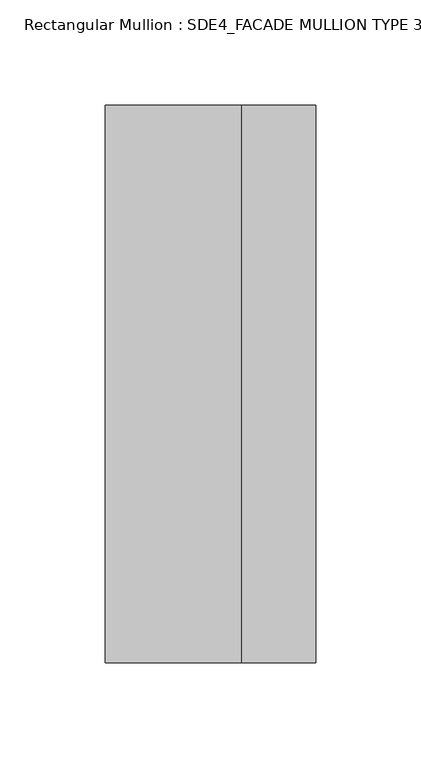
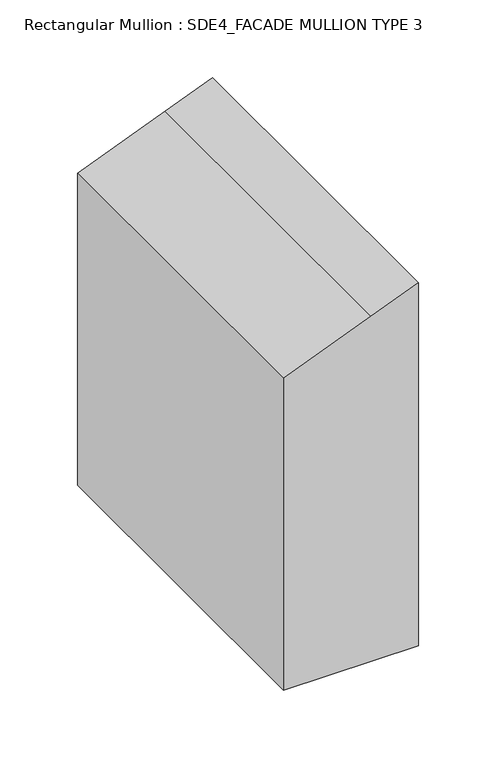
"""IFC4 building model written with IfcOpenShell, lengths in millimetres: member geometry, Rectangular Mullion : SDE4_FACADE MULLION TYPE 3."""

from ifc_helpers import new_model, si_unit, frame, origin, place, context, project, spatial, polyline, outline, extrude, source, transform, mapped, element, save


def rectangular_mullion_sde4_facade_mullion_type_3_aae3be0e(model_context):
    return source(origin(), model_context, "Body", "SweptSolid", [
        extrude(outline(polyline([(-23.0813185, 50.0), (-37.1390676, 14.8556271), (-63.0813185, -50.0), (-307.974544, -50.0), (-307.974544, 50.0), (-23.0813185, 50.0)])), frame((0.0, -132.5, 0.0), z_axis=(0.0, 1.0, 0.0), x_axis=(0.0, 0.0, 1.0)), (0.0, 0.0, 1.0), 265.0),
    ])


if __name__ == "__main__":
    model = new_model("IFC4")
    model_context = context("Model", 3, world=origin())
    ifc_project = project(units=[si_unit("LENGTHUNIT", "METRE", prefix="MILLI")], contexts=[model_context])
    site = spatial("IfcSite", under=ifc_project)
    building = spatial("IfcBuilding", under=site)
    placement = place(None, origin())
    rectangular_mullion_sde4_facade_mullion_type_3_shape = rectangular_mullion_sde4_facade_mullion_type_3_aae3be0e(model_context)
    element("IfcMember", 1, ObjectType="Rectangular Mullion : SDE4_FACADE MULLION TYPE 3", at=placement, inside=building, context=model_context, shape_type="MappedRepresentation", body=[
        mapped(rectangular_mullion_sde4_facade_mullion_type_3_shape, transform((0.0, 0.0, 0.0), x_axis=(1.0, 0.0, 0.0), y_axis=(0.0, 1.0, 0.0), z_axis=(0.0, 0.0, 1.0))),
    ])
    save(model, "model.ifc")

# Revit data of these elements
# Type "Rectangular Mullion : SDE4_FACADE MULLION TYPE 3"
#   built-in parameter 1007322 = 0.869423 (stored number, unit not read)
#   built-in parameter 1007321 = 0.164042 (stored number, unit not read)
#   built-in parameter 1007320 = 0.164042 (stored number, unit not read)
